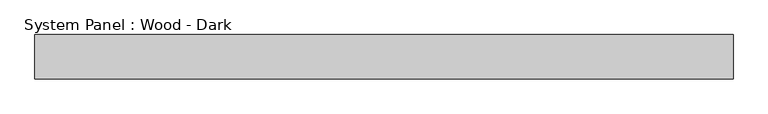
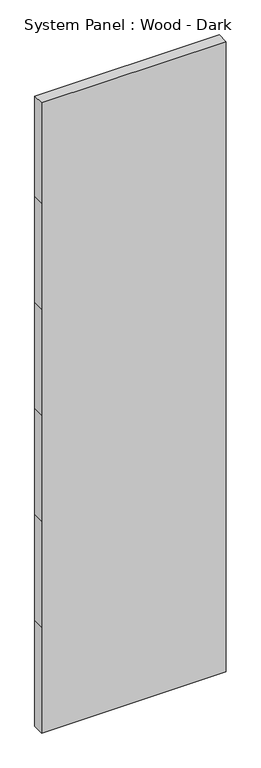
"""IFC4 building model written with IfcOpenShell, lengths in millimetres: plate geometry, System Panel : Wood - Dark."""

import ifcopenshell
import ifcopenshell.guid

model = None  # the IFC model being written
_history = None  # IfcOwnerHistory: only IFC2X3 demands one
_inside = {}  # id of a spatial element -> (the spatial element, [elements in it])
_under = {}  # id of a project, library or spatial element -> (it, [spatial elements below it])
_declared = {}  # id of a project -> (the project, [libraries it declares])
_typed = {}  # id of a type object -> (the type object, [elements of that type])
_made_of = {}  # id of a material, layer set ... -> (it, [elements and type objects made of it])


def new_model(schema):
    """Start an empty IFC model of exactly this schema.

    Asked for "IFC4X3", IfcOpenShell would pick the latest addendum, in which some entities
    have other attributes; the version numbers below select the first issue.
    IFC2X3 requires an IfcOwnerHistory on every rooted entity: one is made here for all.
    """
    global model, _history
    if schema == "IFC4X3":
        model = ifcopenshell.file(schema_version=(4, 3, 0, 0))
    else:
        model = ifcopenshell.file(schema=schema)
    _inside.clear()
    _under.clear()
    _declared.clear()
    _typed.clear()
    _made_of.clear()
    _history = None
    if model.schema == "IFC2X3":
        org = make("IfcOrganization", Name="unknown")
        user = make(
            "IfcPersonAndOrganization",
            ThePerson=make("IfcPerson", FamilyName="unknown"),
            TheOrganization=org,
        )
        app = make(
            "IfcApplication",
            ApplicationDeveloper=org,
            Version="unknown",
            ApplicationFullName="unknown",
            ApplicationIdentifier="unknown",
        )
        _history = make(
            "IfcOwnerHistory",
            OwningUser=user,
            OwningApplication=app,
            ChangeAction="ADDED",
            CreationDate=0,
        )
    return model


def make(cls, **values):
    """One entity of the class cls with the attributes given. An attribute that is None is left unset."""
    return model.create_entity(
        cls, **{name: value for name, value in values.items() if value is not None}
    )


def rooted(cls, **values):
    """An entity with a GlobalId (a new one), such as an element, a storey or a relation."""
    return make(cls, GlobalId=ifcopenshell.guid.new(), OwnerHistory=_history, **values)


def si_unit(unit_type, name, prefix=None):
    """IfcSIUnit, for example si_unit("LENGTHUNIT", "METRE", prefix="MILLI")."""
    return make("IfcSIUnit", UnitType=unit_type, Prefix=prefix, Name=name)


def assignment(units):
    """IfcUnitAssignment: the units of a project."""
    return None if units is None else make("IfcUnitAssignment", Units=units)


def point(xyz):
    """IfcCartesianPoint."""
    return None if xyz is None else make("IfcCartesianPoint", Coordinates=xyz)


def direction(xyz):
    """IfcDirection."""
    return None if xyz is None else make("IfcDirection", DirectionRatios=xyz)


def frame(location, z_axis=None, x_axis=None):
    """IfcAxis2Placement3D, a coordinate frame: its origin and axes. An axis left out is left unset."""
    return make(
        "IfcAxis2Placement3D",
        Location=point(location),
        Axis=direction(z_axis),
        RefDirection=direction(x_axis),
    )


def origin():
    """The frame at (0, 0, 0) with its axes left unset."""
    return frame((0.0, 0.0, 0.0))


def place(relative_to, where):
    """IfcLocalPlacement: puts the frame where relative to a parent placement (None: the world)."""
    return make(
        "IfcLocalPlacement", PlacementRelTo=relative_to, RelativePlacement=where
    )


def context(
    kind, dimensions, precision=None, world=None, true_north=None, identifier=None
):
    """IfcGeometricRepresentationContext, for example the 3D "Model" context."""
    return make(
        "IfcGeometricRepresentationContext",
        ContextIdentifier=identifier,
        ContextType=kind,
        CoordinateSpaceDimension=dimensions,
        Precision=precision,
        WorldCoordinateSystem=world,
        TrueNorth=true_north,
    )


def project(units=None, contexts=None):
    """IfcProject with its units and contexts."""
    return rooted(
        "IfcProject",
        Name="project",
        RepresentationContexts=contexts,
        UnitsInContext=assignment(units),
    )


def spatial(cls, under=None, at=None, **own):
    """A site, building, storey or space (cls), placed at a placement, below another one or the project."""
    s = rooted(cls, ObjectPlacement=at, **own)
    if under is not None:
        _under.setdefault(under.id(), (under, []))[1].append(s)
    return s


def polyline(points):
    """IfcPolyline through the points."""
    return make("IfcPolyline", Points=[point(p) for p in points])


def outline(outer, holes=None, kind="AREA"):
    """IfcArbitraryClosedProfileDef: a profile drawn as a closed curve; with holes, ...WithVoids."""
    if holes is None:
        return make("IfcArbitraryClosedProfileDef", ProfileType=kind, OuterCurve=outer)
    return make(
        "IfcArbitraryProfileDefWithVoids",
        ProfileType=kind,
        OuterCurve=outer,
        InnerCurves=holes,
    )


def extrude(swept, where, along, depth):
    """IfcExtrudedAreaSolid: the profile swept, set in the frame where, extruded along a direction by depth."""
    return make(
        "IfcExtrudedAreaSolid",
        SweptArea=swept,
        Position=where,
        ExtrudedDirection=direction(along),
        Depth=depth,
    )


def shape(context_of_items, identifier, shape_type, items):
    """IfcShapeRepresentation: the items that make up one representation, for example the "Body"."""
    return make(
        "IfcShapeRepresentation",
        ContextOfItems=context_of_items,
        RepresentationIdentifier=identifier,
        RepresentationType=shape_type,
        Items=items,
    )


def source(mapping_origin, context_of_items, identifier, shape_type, items):
    """IfcRepresentationMap: a shape defined once, which mapped items show again and again."""
    return make(
        "IfcRepresentationMap",
        MappingOrigin=mapping_origin,
        MappedRepresentation=shape(context_of_items, identifier, shape_type, items),
    )


def transform(
    local_origin,
    x_axis=None,
    y_axis=None,
    z_axis=None,
    scale=None,
    scale2=None,
    scale3=None,
    uniform=True,
):
    """IfcCartesianTransformationOperator3D, or its non-uniform kind. x_axis, y_axis, z_axis: its Axis1, 2, 3."""
    if uniform:
        return make(
            "IfcCartesianTransformationOperator3D",
            Axis1=direction(x_axis),
            Axis2=direction(y_axis),
            LocalOrigin=point(local_origin),
            Scale=scale,
            Axis3=direction(z_axis),
        )
    return make(
        "IfcCartesianTransformationOperator3DnonUniform",
        Axis1=direction(x_axis),
        Axis2=direction(y_axis),
        LocalOrigin=point(local_origin),
        Scale=scale,
        Axis3=direction(z_axis),
        Scale2=scale2,
        Scale3=scale3,
    )


def mapped(mapping_source, mapping_target):
    """IfcMappedItem: shows the shape of a source again, moved by a transform."""
    return make(
        "IfcMappedItem", MappingSource=mapping_source, MappingTarget=mapping_target
    )


def made_of(thing, what):
    """Note that an element or type object is made of a material, layer set ...; save() writes the relation."""
    if what is not None:
        _made_of.setdefault(what.id(), (what, []))[1].append(thing)
    return thing


def element(
    cls,
    number,
    at=None,
    inside=None,
    cuts=None,
    type_object=None,
    material=None,
    context=None,
    identifier="Body",
    shape_type=None,
    held_by="IfcProductDefinitionShape",
    body=None,
    shapes=None,
    **own,
):
    """One element of the class cls, such as IfcWall. Its Tag is "e" and its number.

    at: its placement. inside: the storey or other place that contains it. cuts: it is an
    opening in that element (IfcRelVoidsElement). A single representation is given by context,
    identifier, shape_type and body (its items); several are given by shapes. held_by: the class
    of the entity that holds the representations. save() writes the other relations.
    """
    e = rooted(cls, Tag="e%d" % number, ObjectPlacement=at, **own)
    if body is not None:
        shapes = [shape(context, identifier, shape_type, body)]
    if shapes is not None:
        e.Representation = make(held_by, Representations=shapes)
    if inside is not None:
        _inside.setdefault(inside.id(), (inside, []))[1].append(e)
    if cuts is not None:
        rooted(
            "IfcRelVoidsElement", RelatingBuildingElement=cuts, RelatedOpeningElement=e
        )
    if type_object is not None:
        _typed.setdefault(type_object.id(), (type_object, []))[1].append(e)
    return made_of(e, material)


def aggregate(whole, parts):
    """IfcRelAggregates: a whole, such as a stair, and the parts it consists of."""
    return rooted("IfcRelAggregates", RelatingObject=whole, RelatedObjects=parts)


def save(model, path):
    """Write the relations noted so far, then the file.

    IfcRelAggregates (storeys below a building ...), IfcRelContainedInSpatialStructure (elements
    in a storey), IfcRelDefinesByType, IfcRelAssociatesMaterial and IfcRelDeclares: one each for
    every whole, place, type object, material and project.
    """
    for whole, parts in _under.values():
        aggregate(whole, parts)
    for where, things in _inside.values():
        rooted(
            "IfcRelContainedInSpatialStructure",
            RelatedElements=things,
            RelatingStructure=where,
        )
    for kind, things in _typed.values():
        rooted("IfcRelDefinesByType", RelatedObjects=things, RelatingType=kind)
    for what, things in _made_of.values():
        rooted("IfcRelAssociatesMaterial", RelatedObjects=things, RelatingMaterial=what)
    for by, libraries in _declared.values():
        rooted("IfcRelDeclares", RelatingContext=by, RelatedDefinitions=libraries)
    model.write(path)


def system_panel_wood_dark_5b9edb8d(model_context):
    return source(origin(), model_context, "Body", "SweptSolid", [
        extrude(outline(polyline([(0.0, -502.1791667), (0.0, 502.1791667), (609.6, 502.1791667), (1219.2, 502.1791667), (1828.8, 502.1791667), (2438.4, 502.1791667), (3048.0, 502.1791667), (3625.85, 502.1791667), (3625.85, -502.1791667), (3048.0, -502.1791667), (2438.4, -502.1791667), (1828.8, -502.1791667), (1219.2, -502.1791667), (609.6, -502.1791667), (0.0, -502.1791667)])), frame((0.0, -19.05, 0.0), z_axis=(0.0, 1.0, 0.0), x_axis=(0.0, 0.0, 1.0)), (0.0, 0.0, 1.0), 63.5),
    ])


if __name__ == "__main__":
    model = new_model("IFC4")
    model_context = context("Model", 3, world=origin())
    ifc_project = project(units=[si_unit("LENGTHUNIT", "METRE", prefix="MILLI")], contexts=[model_context])
    site = spatial("IfcSite", under=ifc_project)
    building = spatial("IfcBuilding", under=site)
    placement = place(None, origin())
    system_panel_wood_dark_shape = system_panel_wood_dark_5b9edb8d(model_context)
    element("IfcPlate", 1, ObjectType="System Panel : Wood - Dark", at=placement, inside=building, context=model_context, shape_type="MappedRepresentation", body=[
        mapped(system_panel_wood_dark_shape, transform((0.0, 0.0, 0.0), x_axis=(1.0, 0.0, 0.0), y_axis=(0.0, 1.0, 0.0), z_axis=(0.0, 0.0, 1.0))),
    ])
    save(model, "model.ifc")

# Revit data of these elements
# Element 1 (IfcPlate, "System Panel : Wood - Dark")
#   Materials on its faces: "Wood Panel - Dark"
# Materials
#   "Wood Panel - Dark": class "Unassigned", colour RGB 57 19 6, transparency 0
